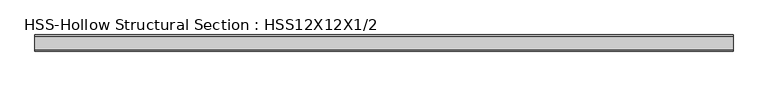
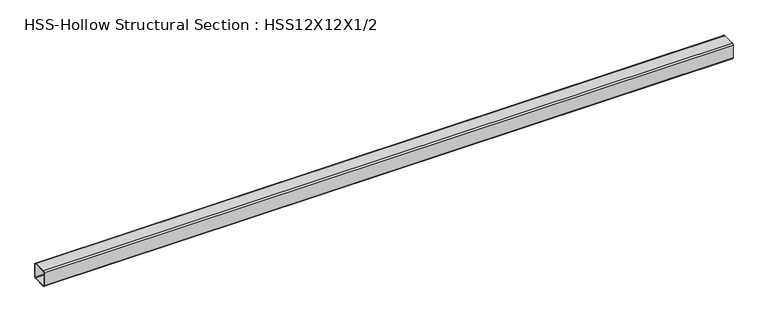
"""IFC4 building model written with IfcOpenShell, lengths in millimetres: beam geometry, HSS-Hollow Structural Section : HSS12X12X1/2."""

import ifcopenshell
import ifcopenshell.guid

model = None  # the IFC model being written
_history = None  # IfcOwnerHistory: only IFC2X3 demands one
_inside = {}  # id of a spatial element -> (the spatial element, [elements in it])
_under = {}  # id of a project, library or spatial element -> (it, [spatial elements below it])
_declared = {}  # id of a project -> (the project, [libraries it declares])
_typed = {}  # id of a type object -> (the type object, [elements of that type])
_made_of = {}  # id of a material, layer set ... -> (it, [elements and type objects made of it])


def new_model(schema):
    """Start an empty IFC model of exactly this schema.

    Asked for "IFC4X3", IfcOpenShell would pick the latest addendum, in which some entities
    have other attributes; the version numbers below select the first issue.
    IFC2X3 requires an IfcOwnerHistory on every rooted entity: one is made here for all.
    """
    global model, _history
    if schema == "IFC4X3":
        model = ifcopenshell.file(schema_version=(4, 3, 0, 0))
    else:
        model = ifcopenshell.file(schema=schema)
    _inside.clear()
    _under.clear()
    _declared.clear()
    _typed.clear()
    _made_of.clear()
    _history = None
    if model.schema == "IFC2X3":
        org = make("IfcOrganization", Name="unknown")
        user = make(
            "IfcPersonAndOrganization",
            ThePerson=make("IfcPerson", FamilyName="unknown"),
            TheOrganization=org,
        )
        app = make(
            "IfcApplication",
            ApplicationDeveloper=org,
            Version="unknown",
            ApplicationFullName="unknown",
            ApplicationIdentifier="unknown",
        )
        _history = make(
            "IfcOwnerHistory",
            OwningUser=user,
            OwningApplication=app,
            ChangeAction="ADDED",
            CreationDate=0,
        )
    return model


def make(cls, **values):
    """One entity of the class cls with the attributes given. An attribute that is None is left unset."""
    return model.create_entity(
        cls, **{name: value for name, value in values.items() if value is not None}
    )


def rooted(cls, **values):
    """An entity with a GlobalId (a new one), such as an element, a storey or a relation."""
    return make(cls, GlobalId=ifcopenshell.guid.new(), OwnerHistory=_history, **values)


def si_unit(unit_type, name, prefix=None):
    """IfcSIUnit, for example si_unit("LENGTHUNIT", "METRE", prefix="MILLI")."""
    return make("IfcSIUnit", UnitType=unit_type, Prefix=prefix, Name=name)


def assignment(units):
    """IfcUnitAssignment: the units of a project."""
    return None if units is None else make("IfcUnitAssignment", Units=units)


def point(xyz):
    """IfcCartesianPoint."""
    return None if xyz is None else make("IfcCartesianPoint", Coordinates=xyz)


def direction(xyz):
    """IfcDirection."""
    return None if xyz is None else make("IfcDirection", DirectionRatios=xyz)


def frame(location, z_axis=None, x_axis=None):
    """IfcAxis2Placement3D, a coordinate frame: its origin and axes. An axis left out is left unset."""
    return make(
        "IfcAxis2Placement3D",
        Location=point(location),
        Axis=direction(z_axis),
        RefDirection=direction(x_axis),
    )


def frame_2d(location, x_axis=None):
    """IfcAxis2Placement2D, a coordinate frame in the plane: its origin and x axis."""
    return make(
        "IfcAxis2Placement2D", Location=point(location), RefDirection=direction(x_axis)
    )


def origin():
    """The frame at (0, 0, 0) with its axes left unset."""
    return frame((0.0, 0.0, 0.0))


def place(relative_to, where):
    """IfcLocalPlacement: puts the frame where relative to a parent placement (None: the world)."""
    return make(
        "IfcLocalPlacement", PlacementRelTo=relative_to, RelativePlacement=where
    )


def context(
    kind, dimensions, precision=None, world=None, true_north=None, identifier=None
):
    """IfcGeometricRepresentationContext, for example the 3D "Model" context."""
    return make(
        "IfcGeometricRepresentationContext",
        ContextIdentifier=identifier,
        ContextType=kind,
        CoordinateSpaceDimension=dimensions,
        Precision=precision,
        WorldCoordinateSystem=world,
        TrueNorth=true_north,
    )


def project(units=None, contexts=None):
    """IfcProject with its units and contexts."""
    return rooted(
        "IfcProject",
        Name="project",
        RepresentationContexts=contexts,
        UnitsInContext=assignment(units),
    )


def spatial(cls, under=None, at=None, **own):
    """A site, building, storey or space (cls), placed at a placement, below another one or the project."""
    s = rooted(cls, ObjectPlacement=at, **own)
    if under is not None:
        _under.setdefault(under.id(), (under, []))[1].append(s)
    return s


def polyline(points):
    """IfcPolyline through the points."""
    return make("IfcPolyline", Points=[point(p) for p in points])


def circle_curve(where, radius):
    """IfcCircle in the frame where."""
    return make("IfcCircle", Position=where, Radius=radius)


def trimmed(basis, trim1, trim2, sense, master):
    """IfcTrimmedCurve: the piece of a basis curve between two trims."""
    return make(
        "IfcTrimmedCurve",
        BasisCurve=basis,
        Trim1=trim1,
        Trim2=trim2,
        SenseAgreement=sense,
        MasterRepresentation=master,
    )


def segment(curve, same_sense, transition):
    """IfcCompositeCurveSegment."""
    return make(
        "IfcCompositeCurveSegment",
        Transition=transition,
        SameSense=same_sense,
        ParentCurve=curve,
    )


def composite_curve(segments, self_intersect=None):
    """IfcCompositeCurve: segments joined end to end."""
    return make("IfcCompositeCurve", Segments=segments, SelfIntersect=self_intersect)


def outline(outer, holes=None, kind="AREA"):
    """IfcArbitraryClosedProfileDef: a profile drawn as a closed curve; with holes, ...WithVoids."""
    if holes is None:
        return make("IfcArbitraryClosedProfileDef", ProfileType=kind, OuterCurve=outer)
    return make(
        "IfcArbitraryProfileDefWithVoids",
        ProfileType=kind,
        OuterCurve=outer,
        InnerCurves=holes,
    )


def extrude(swept, where, along, depth):
    """IfcExtrudedAreaSolid: the profile swept, set in the frame where, extruded along a direction by depth."""
    return make(
        "IfcExtrudedAreaSolid",
        SweptArea=swept,
        Position=where,
        ExtrudedDirection=direction(along),
        Depth=depth,
    )


def shape(context_of_items, identifier, shape_type, items):
    """IfcShapeRepresentation: the items that make up one representation, for example the "Body"."""
    return make(
        "IfcShapeRepresentation",
        ContextOfItems=context_of_items,
        RepresentationIdentifier=identifier,
        RepresentationType=shape_type,
        Items=items,
    )


def source(mapping_origin, context_of_items, identifier, shape_type, items):
    """IfcRepresentationMap: a shape defined once, which mapped items show again and again."""
    return make(
        "IfcRepresentationMap",
        MappingOrigin=mapping_origin,
        MappedRepresentation=shape(context_of_items, identifier, shape_type, items),
    )


def transform(
    local_origin,
    x_axis=None,
    y_axis=None,
    z_axis=None,
    scale=None,
    scale2=None,
    scale3=None,
    uniform=True,
):
    """IfcCartesianTransformationOperator3D, or its non-uniform kind. x_axis, y_axis, z_axis: its Axis1, 2, 3."""
    if uniform:
        return make(
            "IfcCartesianTransformationOperator3D",
            Axis1=direction(x_axis),
            Axis2=direction(y_axis),
            LocalOrigin=point(local_origin),
            Scale=scale,
            Axis3=direction(z_axis),
        )
    return make(
        "IfcCartesianTransformationOperator3DnonUniform",
        Axis1=direction(x_axis),
        Axis2=direction(y_axis),
        LocalOrigin=point(local_origin),
        Scale=scale,
        Axis3=direction(z_axis),
        Scale2=scale2,
        Scale3=scale3,
    )


def mapped(mapping_source, mapping_target):
    """IfcMappedItem: shows the shape of a source again, moved by a transform."""
    return make(
        "IfcMappedItem", MappingSource=mapping_source, MappingTarget=mapping_target
    )


def made_of(thing, what):
    """Note that an element or type object is made of a material, layer set ...; save() writes the relation."""
    if what is not None:
        _made_of.setdefault(what.id(), (what, []))[1].append(thing)
    return thing


def element(
    cls,
    number,
    at=None,
    inside=None,
    cuts=None,
    type_object=None,
    material=None,
    context=None,
    identifier="Body",
    shape_type=None,
    held_by="IfcProductDefinitionShape",
    body=None,
    shapes=None,
    **own,
):
    """One element of the class cls, such as IfcWall. Its Tag is "e" and its number.

    at: its placement. inside: the storey or other place that contains it. cuts: it is an
    opening in that element (IfcRelVoidsElement). A single representation is given by context,
    identifier, shape_type and body (its items); several are given by shapes. held_by: the class
    of the entity that holds the representations. save() writes the other relations.
    """
    e = rooted(cls, Tag="e%d" % number, ObjectPlacement=at, **own)
    if body is not None:
        shapes = [shape(context, identifier, shape_type, body)]
    if shapes is not None:
        e.Representation = make(held_by, Representations=shapes)
    if inside is not None:
        _inside.setdefault(inside.id(), (inside, []))[1].append(e)
    if cuts is not None:
        rooted(
            "IfcRelVoidsElement", RelatingBuildingElement=cuts, RelatedOpeningElement=e
        )
    if type_object is not None:
        _typed.setdefault(type_object.id(), (type_object, []))[1].append(e)
    return made_of(e, material)


def aggregate(whole, parts):
    """IfcRelAggregates: a whole, such as a stair, and the parts it consists of."""
    return rooted("IfcRelAggregates", RelatingObject=whole, RelatedObjects=parts)


def save(model, path):
    """Write the relations noted so far, then the file.

    IfcRelAggregates (storeys below a building ...), IfcRelContainedInSpatialStructure (elements
    in a storey), IfcRelDefinesByType, IfcRelAssociatesMaterial and IfcRelDeclares: one each for
    every whole, place, type object, material and project.
    """
    for whole, parts in _under.values():
        aggregate(whole, parts)
    for where, things in _inside.values():
        rooted(
            "IfcRelContainedInSpatialStructure",
            RelatedElements=things,
            RelatingStructure=where,
        )
    for kind, things in _typed.values():
        rooted("IfcRelDefinesByType", RelatedObjects=things, RelatingType=kind)
    for what, things in _made_of.values():
        rooted("IfcRelAssociatesMaterial", RelatedObjects=things, RelatingMaterial=what)
    for by, libraries in _declared.values():
        rooted("IfcRelDeclares", RelatingContext=by, RelatedDefinitions=libraries)
    model.write(path)


def hss_hollow_structural_section_hss12x12x1_2_830ae8b1(model_context):
    return source(origin(), model_context, "Body", "SweptSolid", [
        extrude(outline(composite_curve([segment(polyline([(152.4, 128.778), (152.4, -128.778)]), True, "CONTINUOUS"), segment(trimmed(circle_curve(frame_2d((128.778, -128.778)), 23.622), [point((152.4, -128.778))], [point((128.778, -152.4))], False, "CARTESIAN"), True, "CONTINUOUS"), segment(polyline([(128.778, -152.4), (-128.778, -152.4)]), True, "CONTINUOUS"), segment(trimmed(circle_curve(frame_2d((-128.778, -128.778)), 23.622), [point((-128.778, -152.4))], [point((-152.4, -128.778))], False, "CARTESIAN"), True, "CONTINUOUS"), segment(polyline([(-152.4, -128.778), (-152.4, 128.778)]), True, "CONTINUOUS"), segment(trimmed(circle_curve(frame_2d((-128.778, 128.778)), 23.622), [point((-152.4, 128.778))], [point((-128.778, 152.4))], False, "CARTESIAN"), True, "CONTINUOUS"), segment(polyline([(-128.778, 152.4), (128.778, 152.4)]), True, "CONTINUOUS"), segment(trimmed(circle_curve(frame_2d((128.778, 128.778)), 23.622), [point((128.778, 152.4))], [point((152.4, 128.778))], False, "CARTESIAN"), True, "CONTINUOUS")], self_intersect=False), holes=[composite_curve([segment(trimmed(circle_curve(frame_2d((-128.778, 128.778)), 11.811), [point((-128.778, 140.589))], [point((-140.589, 128.778))], True, "CARTESIAN"), True, "CONTINUOUS"), segment(polyline([(-140.589, 128.778), (-140.589, -128.778)]), True, "CONTINUOUS"), segment(trimmed(circle_curve(frame_2d((-128.778, -128.778)), 11.811), [point((-140.589, -128.778))], [point((-128.778, -140.589))], True, "CARTESIAN"), True, "CONTINUOUS"), segment(polyline([(-128.778, -140.589), (128.778, -140.589)]), True, "CONTINUOUS"), segment(trimmed(circle_curve(frame_2d((128.778, -128.778)), 11.811), [point((128.778, -140.589))], [point((140.589, -128.778))], True, "CARTESIAN"), True, "CONTINUOUS"), segment(polyline([(140.589, -128.778), (140.589, 128.778)]), True, "CONTINUOUS"), segment(trimmed(circle_curve(frame_2d((128.778, 128.778)), 11.811), [point((140.589, 128.778))], [point((128.778, 140.589))], True, "CARTESIAN"), True, "CONTINUOUS"), segment(polyline([(128.778, 140.589), (-128.778, 140.589)]), True, "CONTINUOUS")], self_intersect=False)]), frame((-6674.2846052, 0.0, 0.0), z_axis=(1.0, 0.0, 0.0), x_axis=(0.0, 1.0, 0.0)), (0.0, 0.0, 1.0), 13185.2498362),
    ])


if __name__ == "__main__":
    model = new_model("IFC4")
    model_context = context("Model", 3, world=origin())
    ifc_project = project(units=[si_unit("LENGTHUNIT", "METRE", prefix="MILLI")], contexts=[model_context])
    site = spatial("IfcSite", under=ifc_project)
    building = spatial("IfcBuilding", under=site)
    placement = place(None, origin())
    hss_hollow_structural_section_hss12x12x1_2_shape = hss_hollow_structural_section_hss12x12x1_2_830ae8b1(model_context)
    element("IfcBeam", 1, ObjectType="HSS-Hollow Structural Section : HSS12X12X1/2", at=placement, inside=building, context=model_context, shape_type="MappedRepresentation", body=[
        mapped(hss_hollow_structural_section_hss12x12x1_2_shape, transform((0.0, 0.0, 0.0), x_axis=(1.0, 0.0, 0.0), y_axis=(0.0, 1.0, 0.0), z_axis=(0.0, 0.0, 1.0))),
    ])
    save(model, "model.ifc")

# Revit data of these elements
# Type "HSS-Hollow Structural Section : HSS12X12X1/2"
#   Assembly Code = "B10"
#   Shape = "Square"
#   W = 75.9
#   Ht = 304.8 mm
#   Length [instance default] = 1524 mm
#   b = 304.8 mm
#   kr = 23.622 mm
#   t = 11.811 mm
#   A = 0.0134838 m²
#   Structural Material [instance default] = Steel ASTM A500, Grade B, Rectangular and Square
# Element 1 (IfcBeam, "HSS-Hollow Structural Section : HSS12X12X1/2")
#   Structural Material = Aluminum 7175 T73 0 Hot Formed
#   Materials on its faces: "Aluminum 7175 T73 0 Hot Formed"
# Materials
#   "Steel ASTM A500, Grade B, Rectangular and Square": class "Metal", colour RGB 199 199 199, transparency 0, Description = "Carbon steel", Cost = 0
#   "Aluminum 7175 T73 0 Hot Formed": class "Metal", colour RGB 120 120 120, transparency 0, Description = "Physical material.", Cost = 0
